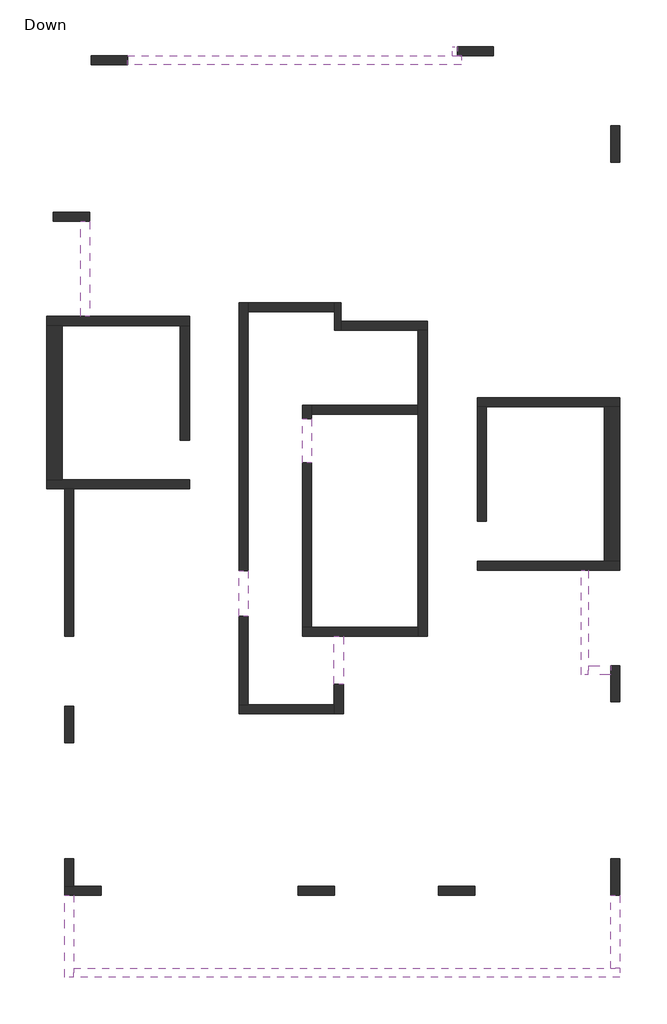
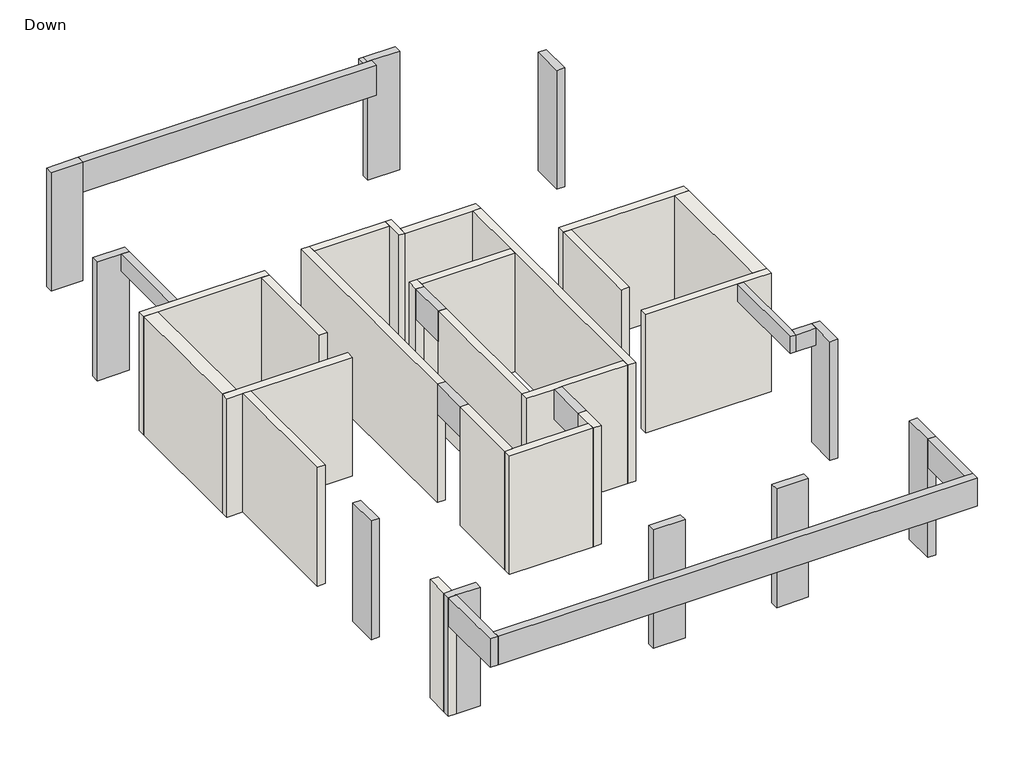
# One storey: 22 walls, 11 beams, 10 columns.
"""IFC4 building model written with IfcOpenShell, lengths in millimetres."""

import ifcopenshell
import ifcopenshell.guid

model = None  # the IFC model being written
_history = None  # IfcOwnerHistory: only IFC2X3 demands one
_inside = {}  # id of a spatial element -> (the spatial element, [elements in it])
_under = {}  # id of a project, library or spatial element -> (it, [spatial elements below it])
_declared = {}  # id of a project -> (the project, [libraries it declares])
_typed = {}  # id of a type object -> (the type object, [elements of that type])
_made_of = {}  # id of a material, layer set ... -> (it, [elements and type objects made of it])


def new_model(schema):
    """Start an empty IFC model of exactly this schema.

    Asked for "IFC4X3", IfcOpenShell would pick the latest addendum, in which some entities
    have other attributes; the version numbers below select the first issue.
    IFC2X3 requires an IfcOwnerHistory on every rooted entity: one is made here for all.
    """
    global model, _history
    if schema == "IFC4X3":
        model = ifcopenshell.file(schema_version=(4, 3, 0, 0))
    else:
        model = ifcopenshell.file(schema=schema)
    _inside.clear()
    _under.clear()
    _declared.clear()
    _typed.clear()
    _made_of.clear()
    _history = None
    if model.schema == "IFC2X3":
        org = make("IfcOrganization", Name="unknown")
        user = make(
            "IfcPersonAndOrganization",
            ThePerson=make("IfcPerson", FamilyName="unknown"),
            TheOrganization=org,
        )
        app = make(
            "IfcApplication",
            ApplicationDeveloper=org,
            Version="unknown",
            ApplicationFullName="unknown",
            ApplicationIdentifier="unknown",
        )
        _history = make(
            "IfcOwnerHistory",
            OwningUser=user,
            OwningApplication=app,
            ChangeAction="ADDED",
            CreationDate=0,
        )
    return model


def make(cls, **values):
    """One entity of the class cls with the attributes given. An attribute that is None is left unset."""
    return model.create_entity(
        cls, **{name: value for name, value in values.items() if value is not None}
    )


def rooted(cls, **values):
    """An entity with a GlobalId (a new one), such as an element, a storey or a relation."""
    return make(cls, GlobalId=ifcopenshell.guid.new(), OwnerHistory=_history, **values)


def si_unit(unit_type, name, prefix=None):
    """IfcSIUnit, for example si_unit("LENGTHUNIT", "METRE", prefix="MILLI")."""
    return make("IfcSIUnit", UnitType=unit_type, Prefix=prefix, Name=name)


def assignment(units):
    """IfcUnitAssignment: the units of a project."""
    return None if units is None else make("IfcUnitAssignment", Units=units)


def point(xyz):
    """IfcCartesianPoint."""
    return None if xyz is None else make("IfcCartesianPoint", Coordinates=xyz)


def direction(xyz):
    """IfcDirection."""
    return None if xyz is None else make("IfcDirection", DirectionRatios=xyz)


def frame(location, z_axis=None, x_axis=None):
    """IfcAxis2Placement3D, a coordinate frame: its origin and axes. An axis left out is left unset."""
    return make(
        "IfcAxis2Placement3D",
        Location=point(location),
        Axis=direction(z_axis),
        RefDirection=direction(x_axis),
    )


def origin():
    """The frame at (0, 0, 0) with its axes left unset."""
    return frame((0.0, 0.0, 0.0))


def place(relative_to, where):
    """IfcLocalPlacement: puts the frame where relative to a parent placement (None: the world)."""
    return make(
        "IfcLocalPlacement", PlacementRelTo=relative_to, RelativePlacement=where
    )


def context(
    kind, dimensions, precision=None, world=None, true_north=None, identifier=None
):
    """IfcGeometricRepresentationContext, for example the 3D "Model" context."""
    return make(
        "IfcGeometricRepresentationContext",
        ContextIdentifier=identifier,
        ContextType=kind,
        CoordinateSpaceDimension=dimensions,
        Precision=precision,
        WorldCoordinateSystem=world,
        TrueNorth=true_north,
    )


def project(units=None, contexts=None):
    """IfcProject with its units and contexts."""
    return rooted(
        "IfcProject",
        Name="project",
        RepresentationContexts=contexts,
        UnitsInContext=assignment(units),
    )


def spatial(cls, under=None, at=None, **own):
    """A site, building, storey or space (cls), placed at a placement, below another one or the project."""
    s = rooted(cls, ObjectPlacement=at, **own)
    if under is not None:
        _under.setdefault(under.id(), (under, []))[1].append(s)
    return s


def polyline(points):
    """IfcPolyline through the points."""
    return make("IfcPolyline", Points=[point(p) for p in points])


def outline(outer, holes=None, kind="AREA"):
    """IfcArbitraryClosedProfileDef: a profile drawn as a closed curve; with holes, ...WithVoids."""
    if holes is None:
        return make("IfcArbitraryClosedProfileDef", ProfileType=kind, OuterCurve=outer)
    return make(
        "IfcArbitraryProfileDefWithVoids",
        ProfileType=kind,
        OuterCurve=outer,
        InnerCurves=holes,
    )


def extrude(swept, where, along, depth):
    """IfcExtrudedAreaSolid: the profile swept, set in the frame where, extruded along a direction by depth."""
    return make(
        "IfcExtrudedAreaSolid",
        SweptArea=swept,
        Position=where,
        ExtrudedDirection=direction(along),
        Depth=depth,
    )


def faces_of(points, faces, orient=None, outer=None):
    """IfcFace entities. A face is a list of loops; a loop is a list of indices into points, from 0.

    orient and outer hold one flag for each loop. By default every Orientation is true, the
    first loop of a face is its IfcFaceOuterBound and the others are IfcFaceBound.
    """
    made = []
    for i, loops in enumerate(faces):
        bounds = []
        for j, loop in enumerate(loops):
            is_outer = j == 0 if outer is None else outer[i][j]
            bounds.append(
                make(
                    "IfcFaceOuterBound" if is_outer else "IfcFaceBound",
                    Bound=make("IfcPolyLoop", Polygon=[points[k] for k in loop]),
                    Orientation=True if orient is None else orient[i][j],
                )
            )
        made.append(make("IfcFace", Bounds=bounds))
    return made


def faceted_brep(points, faces, orient=None, outer=None, voids=None):
    """IfcFacetedBrep: a solid bounded by flat faces; with voids (closed shells), ...WithVoids."""
    shared = [point(p) for p in points]
    hull = make("IfcClosedShell", CfsFaces=faces_of(shared, faces, orient, outer))
    if voids is None:
        return make("IfcFacetedBrep", Outer=hull)
    return make(
        "IfcFacetedBrepWithVoids",
        Outer=hull,
        Voids=[
            make(cls, CfsFaces=faces_of(shared, fs, o, b)) for cls, fs, o, b in voids
        ],
    )


def shape(context_of_items, identifier, shape_type, items):
    """IfcShapeRepresentation: the items that make up one representation, for example the "Body"."""
    return make(
        "IfcShapeRepresentation",
        ContextOfItems=context_of_items,
        RepresentationIdentifier=identifier,
        RepresentationType=shape_type,
        Items=items,
    )


def made_of(thing, what):
    """Note that an element or type object is made of a material, layer set ...; save() writes the relation."""
    if what is not None:
        _made_of.setdefault(what.id(), (what, []))[1].append(thing)
    return thing


def element(
    cls,
    number,
    at=None,
    inside=None,
    cuts=None,
    type_object=None,
    material=None,
    context=None,
    identifier="Body",
    shape_type=None,
    held_by="IfcProductDefinitionShape",
    body=None,
    shapes=None,
    **own,
):
    """One element of the class cls, such as IfcWall. Its Tag is "e" and its number.

    at: its placement. inside: the storey or other place that contains it. cuts: it is an
    opening in that element (IfcRelVoidsElement). A single representation is given by context,
    identifier, shape_type and body (its items); several are given by shapes. held_by: the class
    of the entity that holds the representations. save() writes the other relations.
    """
    e = rooted(cls, Tag="e%d" % number, ObjectPlacement=at, **own)
    if body is not None:
        shapes = [shape(context, identifier, shape_type, body)]
    if shapes is not None:
        e.Representation = make(held_by, Representations=shapes)
    if inside is not None:
        _inside.setdefault(inside.id(), (inside, []))[1].append(e)
    if cuts is not None:
        rooted(
            "IfcRelVoidsElement", RelatingBuildingElement=cuts, RelatedOpeningElement=e
        )
    if type_object is not None:
        _typed.setdefault(type_object.id(), (type_object, []))[1].append(e)
    return made_of(e, material)


def aggregate(whole, parts):
    """IfcRelAggregates: a whole, such as a stair, and the parts it consists of."""
    return rooted("IfcRelAggregates", RelatingObject=whole, RelatedObjects=parts)


def save(model, path):
    """Write the relations noted so far, then the file.

    IfcRelAggregates (storeys below a building ...), IfcRelContainedInSpatialStructure (elements
    in a storey), IfcRelDefinesByType, IfcRelAssociatesMaterial and IfcRelDeclares: one each for
    every whole, place, type object, material and project.
    """
    for whole, parts in _under.values():
        aggregate(whole, parts)
    for where, things in _inside.values():
        rooted(
            "IfcRelContainedInSpatialStructure",
            RelatedElements=things,
            RelatingStructure=where,
        )
    for kind, things in _typed.values():
        rooted("IfcRelDefinesByType", RelatedObjects=things, RelatingType=kind)
    for what, things in _made_of.values():
        rooted("IfcRelAssociatesMaterial", RelatedObjects=things, RelatingMaterial=what)
    for by, libraries in _declared.values():
        rooted("IfcRelDeclares", RelatingContext=by, RelatedDefinitions=libraries)
    model.write(path)


model = new_model("IFC4")

# Units and contexts
model_context = context("Model", 3, world=origin())
ifc_project = project(units=[si_unit("LENGTHUNIT", "METRE", prefix="MILLI")], contexts=[model_context])

# Site, building, storey
site = spatial("IfcSite", under=ifc_project)
building = spatial("IfcBuilding", under=site)
storey = spatial("IfcBuildingStorey", under=building, Name="Down", Elevation=0.0)

# Beams
placement = place(None, origin())
element("IfcBeam", 1, ObjectType="Concrete Rectengular Beam : 15/45", at=placement, inside=storey, context=model_context, shape_type="Brep", body=[
    faceted_brep([(-8943.1419846, 24273.2318976, 3150.0), (-9093.1419846, 24273.2318976, 3150.0), (-9093.1419846, 21971.29434, 3150.0), (-8943.1419846, 21971.29434, 3150.0), (-8943.1419846, 22171.29434, 3150.0), (-9093.1419846, 24273.2318976, 2920.0), (-9093.1419846, 24273.2318976, 2700.0), (-9093.1419846, 21971.29434, 2700.0), (-9093.1419846, 21971.29434, 2920.0), (-8943.1419846, 24273.2318976, 2700.0), (-8943.1419846, 22171.4624057, 2700.0), (-8943.1419846, 22171.29434, 2700.0), (-8943.1419846, 21971.29434, 2700.0), (-8943.1419846, 24273.2318976, 2850.0), (-8943.1419846, 21971.29434, 2920.0)], [[[0, 1, 2, 3, 4]], [[2, 1, 5, 6, 7, 8]], [[6, 9, 10, 11, 12, 7]], [[9, 13, 0, 4, 3, 14, 12, 11, 10]], [[1, 0, 13, 9, 6, 5]], [[3, 2, 8, 7, 12, 14]]]),
])
element("IfcBeam", 2, ObjectType="Concrete Rectengular Beam : 20/45", at=placement, inside=storey, context=model_context, shape_type="Brep", body=[
    faceted_brep([(-19934.1305711, 31959.1185492, 3150.0), (-20134.1305711, 31959.1185492, 3150.0), (-20134.1305711, 29864.251036, 3150.0), (-19934.1305711, 29864.251036, 3150.0), (-20134.1305711, 31959.1185492, 2850.0), (-20134.1305711, 31959.1185492, 2700.0), (-20134.1305711, 29864.251036, 2700.0), (-20134.1305711, 29864.251036, 2850.0), (-19934.1305711, 31959.1185492, 2700.0), (-19934.1305711, 29864.251036, 2700.0), (-19934.1305711, 29864.251036, 2920.0), (-19934.1305711, 31959.1185492, 2920.0)], [[[0, 1, 2, 3]], [[1, 4, 5, 6, 7, 2]], [[5, 8, 9, 6]], [[0, 3, 10, 9, 8, 11]], [[1, 0, 11, 8, 5, 4]], [[3, 2, 7, 6, 9, 10]]]),
])
element("IfcBeam", 3, ObjectType="Concrete Rectengular Beam : 20/45", at=placement, inside=storey, context=model_context, shape_type="Brep", body=[
    faceted_brep([(-8445.045869, 21971.29434, 3150.0), (-8445.045869, 22171.29434, 3150.0), (-8943.1419846, 22171.29434, 3150.0), (-8943.1419846, 21971.29434, 3150.0), (-8445.045869, 22171.29434, 2700.0), (-8943.1419846, 22171.29434, 2700.0), (-8445.045869, 21971.29434, 2700.0), (-8943.1419846, 21971.29434, 2700.0), (-8445.045869, 21971.29434, 2920.0)], [[[0, 1, 2, 3]], [[1, 4, 5, 2]], [[4, 6, 7, 5]], [[6, 8, 0, 3, 7]], [[1, 0, 8, 6, 4]], [[3, 2, 5, 7]]]),
])
element("IfcBeam", 4, ObjectType="Concrete Rectengular Beam : 20/75", at=placement, inside=storey, context=model_context, shape_type="Brep", body=[
    faceted_brep([(-20285.7922608, 17115.8692988, 3150.0), (-20485.7922608, 17115.8692988, 3150.0), (-20485.7922608, 15302.6614945, 3150.0), (-20285.7922608, 15302.6614945, 3150.0), (-20285.7922608, 15502.6614945, 3150.0), (-20485.7922608, 15302.6614945, 2400.0), (-20485.7922608, 17115.8692988, 2400.0), (-20285.7922608, 17115.8692988, 2400.0), (-20285.7922608, 15502.6614945, 2400.0), (-20285.7922608, 15302.6614945, 2400.0), (-20285.7922608, 17115.8692988, 2920.0)], [[[0, 1, 2, 3, 4]], [[5, 2, 1, 6]], [[6, 7, 8, 9, 5]], [[3, 9, 8, 7, 10, 0, 4]], [[1, 0, 10, 7, 6]], [[3, 2, 5, 9]]]),
])
element("IfcBeam", 5, ObjectType="Concrete Rectengular Beam : 20/75", at=placement, inside=storey, context=model_context, shape_type="Brep", body=[
    faceted_brep([(-8245.045869, 15302.6614945, 3150.0), (-8245.045869, 15502.6614945, 3150.0), (-8445.045869, 15502.6614945, 3150.0), (-20285.7922608, 15502.6614945, 3150.0), (-20285.7922608, 15302.6614945, 3150.0), (-8245.045869, 15302.6614945, 2400.0), (-20285.7922608, 15302.6614945, 2400.0), (-8245.045869, 15502.6614945, 2400.0), (-20285.7922608, 15502.6614945, 2400.0), (-8445.045869, 15502.6614945, 2400.0), (-20285.7922608, 15502.6614945, 2920.0)], [[[0, 1, 2, 3, 4]], [[5, 0, 4, 6]], [[7, 5, 6, 8, 9]], [[1, 7, 9, 8, 10, 3, 2]], [[4, 3, 10, 8, 6]], [[1, 0, 5, 7]]]),
])
element("IfcBeam", 6, ObjectType="Concrete Rectengular Beam : 20/75", at=placement, inside=storey, context=model_context, shape_type="Brep", body=[
    faceted_brep([(-8245.045869, 17114.2549976, 3150.0), (-8445.045869, 17114.2549976, 3150.0), (-8445.045869, 15502.6614945, 3150.0), (-8245.045869, 15502.6614945, 3150.0), (-8245.045869, 17114.2549976, 2400.0), (-8245.045869, 15502.6614945, 2400.0), (-8445.045869, 17114.2549976, 2400.0), (-8445.045869, 15502.6614945, 2400.0), (-8445.045869, 17114.2549976, 2920.0), (-8445.045869, 15502.6614945, 2920.0)], [[[0, 1, 2, 3]], [[4, 0, 3, 5]], [[6, 4, 5, 7]], [[2, 1, 8, 6, 7, 9]], [[1, 0, 4, 6, 8]], [[3, 2, 9, 7, 5]]]),
])
element("IfcBeam", 7, ObjectType="Concrete Rectengular Beam : 20/80", at=placement, inside=storey, context=model_context, shape_type="Brep", body=[
    faceted_brep([(-11741.5564046, 35608.8121294, 3150.0), (-11741.5564046, 35408.8121294, 3150.0), (-11741.5564046, 35408.8121294, 2920.0), (-11741.5564046, 35408.8121294, 2350.0), (-11741.5564046, 35608.8121294, 2350.0), (-11741.5564046, 35608.8121294, 2920.0), (-11742.9937266, 35608.8121294, 3150.0), (-11942.9937266, 35608.8121294, 3150.0), (-19101.5564046, 35608.8121294, 3150.0), (-19101.5564046, 35408.8121294, 3150.0), (-19101.5564046, 35408.8121294, 2920.0), (-19101.5564046, 35408.8121294, 2350.0), (-19101.5564046, 35608.8121294, 2350.0), (-11942.9937266, 35608.8121294, 2350.0), (-11742.9937266, 35608.8121294, 2350.0)], [[[0, 1, 2, 3, 4, 5]], [[1, 0, 6, 7, 8, 9]], [[1, 9, 10, 11, 3, 2]], [[4, 3, 11, 12, 13, 14]], [[12, 8, 7, 6, 0, 5, 4, 14, 13]], [[9, 8, 12, 11, 10]]]),
])
element("IfcBeam", 8, ObjectType="Concrete Rectengular Beam : 20/80", at=placement, inside=storey, context=model_context, shape_type="SweptSolid", body=[
    extrude(outline(polyline([(-11833.3239157, 35608.9801951), (-11742.9937266, 35608.9801951), (-11742.9937266, 35608.8121294), (-11942.9937266, 35608.8121294), (-11942.9937266, 35808.8121294), (-11833.3239157, 35808.8121294), (-11833.3239157, 35608.9801951)])), frame((0.0, 0.0, 2350.0), z_axis=(0.0, 0.0, 1.0), x_axis=(1.0, 0.0, 0.0)), (0.0, 0.0, 1.0), 800.0),
])
element("IfcBeam", 9, ObjectType="Concrete Rectengular Beam : 20/80", at=placement, inside=storey, context=model_context, shape_type="Brep", body=[
    faceted_brep([(-16642.902761, 24264.0058702, 3150.0), (-16442.902761, 24264.0058702, 3150.0), (-16442.902761, 24264.0058702, 2350.0), (-16642.902761, 24264.0058702, 2350.0), (-16642.902761, 24264.0058702, 2920.0), (-16642.902761, 23263.128057, 2350.0), (-16442.902761, 23263.128057, 2350.0), (-16442.902761, 23263.128057, 3150.0), (-16642.902761, 23263.128057, 3150.0), (-16642.902761, 23263.128057, 2920.0)], [[[0, 1, 2, 3, 4]], [[5, 6, 7, 8, 9]], [[1, 0, 8, 7]], [[2, 1, 7, 6]], [[3, 2, 6, 5]], [[8, 0, 4, 3, 5, 9]]]),
])
element("IfcBeam", 10, ObjectType="Concrete Rectengular Beam : 20/80", at=placement, inside=storey, context=model_context, shape_type="Brep", body=[
    faceted_brep([(-15041.6888164, 27611.1233031, 2350.0), (-15241.6888164, 27611.1233031, 2350.0), (-15241.6888164, 27611.1233031, 2920.0), (-15241.6888164, 27611.1233031, 3150.0), (-15046.6888164, 27611.1233031, 3150.0), (-15046.6888164, 27611.1233031, 2920.0), (-15041.6888164, 27611.1233031, 2920.0), (-15241.6888164, 26638.171559, 2350.0), (-15041.6888164, 26638.171559, 2350.0), (-15041.6888164, 26638.171559, 2920.0), (-15046.6888164, 26638.171559, 2920.0), (-15046.6888164, 26638.171559, 3150.0), (-15241.6888164, 26638.171559, 3150.0), (-15241.6888164, 26638.171559, 2920.0)], [[[0, 1, 2, 3, 4, 5, 6]], [[7, 8, 9, 10, 11, 12, 13]], [[3, 12, 11, 4]], [[8, 0, 6, 9]], [[1, 0, 8, 7]], [[12, 3, 2, 1, 7, 13]], [[5, 10, 9, 6]], [[10, 5, 4, 11]]]),
])
element("IfcBeam", 11, ObjectType="Concrete Rectengular Beam : 20/80", at=placement, inside=storey, context=model_context, shape_type="Brep", body=[
    faceted_brep([(-14543.2190847, 21764.1541281, 2350.0), (-14343.2190847, 21764.1541281, 2350.0), (-14343.2190847, 21764.1541281, 2920.0), (-14343.2190847, 21764.1541281, 3150.0), (-14543.2190847, 21764.1541281, 3150.0), (-14543.2190847, 21764.1541281, 2920.0), (-14343.2190847, 22813.9119334, 3150.0), (-14543.2190847, 22813.9119334, 3150.0), (-14343.2190847, 22813.9119334, 2350.0), (-14343.2190847, 22813.9119334, 2920.0), (-14543.2190847, 22813.9119334, 2350.0), (-14543.2190847, 22813.9119334, 2920.0)], [[[0, 1, 2, 3, 4, 5]], [[4, 3, 6, 7]], [[6, 3, 2, 1, 8, 9]], [[1, 0, 10, 8]], [[4, 7, 11, 10, 0, 5]], [[7, 6, 9, 8, 10, 11]]]),
])

# Columns
element("IfcColumn", 12, ObjectType="Concrete Rectengular Column : 20/80", at=placement, inside=storey, context=model_context, shape_type="Brep", body=[
    faceted_brep([(-19901.5564046, 35608.8121294, 0.0), (-19101.5564046, 35608.8121294, 0.0), (-19101.5564046, 35408.8121294, 0.0), (-19901.5564046, 35408.8121294, 0.0), (-19901.5564046, 35608.8121294, 3150.0), (-19101.5564046, 35608.8121294, 3150.0), (-19901.5564046, 35608.8121294, 2920.0), (-19101.5564046, 35408.8121294, 3150.0), (-19901.5564046, 35408.8121294, 3150.0), (-19901.5564046, 35408.8121294, 2920.0)], [[[0, 1, 2, 3]], [[4, 5, 1, 0, 6]], [[5, 7, 2, 1]], [[7, 8, 9, 3, 2]], [[8, 4, 6, 0, 3, 9]], [[4, 8, 7, 5]]]),
])
element("IfcColumn", 13, ObjectType="Concrete Rectengular Column : 20/80", at=placement, inside=storey, context=model_context, shape_type="Brep", body=[
    faceted_brep([(-11833.3239157, 35808.9801951, 0.0), (-11033.3239157, 35808.9801951, 0.0), (-11033.3239157, 35608.9801951, 0.0), (-11833.3239157, 35608.9801951, 0.0), (-11833.3239157, 35808.9801951, 3150.0), (-11033.3239157, 35808.9801951, 3150.0), (-11033.3239157, 35808.9801951, 2920.0), (-11033.3239157, 35608.9801951, 3150.0), (-11033.3239157, 35608.9801951, 2920.0), (-11741.5564046, 35608.9801951, 3150.0), (-11833.3239157, 35608.9801951, 3150.0)], [[[0, 1, 2, 3]], [[4, 5, 6, 1, 0]], [[5, 7, 8, 2, 1, 6]], [[7, 9, 10, 3, 2, 8]], [[10, 4, 0, 3]], [[4, 10, 9, 7, 5]]]),
])
element("IfcColumn", 14, ObjectType="Concrete Rectengular Column : 20/80", at=placement, inside=storey, context=model_context, shape_type="Brep", body=[
    faceted_brep([(-8445.045869, 33260.248461, 0.0), (-8445.045869, 34060.248461, 0.0), (-8245.045869, 34060.248461, 0.0), (-8245.045869, 33260.248461, 0.0), (-8445.045869, 33260.248461, 3150.0), (-8445.045869, 34060.248461, 3150.0), (-8445.045869, 34060.248461, 2920.0), (-8445.045869, 33260.248461, 2920.0), (-8245.045869, 34060.248461, 3150.0), (-8245.045869, 34060.248461, 2920.0), (-8245.045869, 33260.248461, 3150.0), (-8245.045869, 33260.248461, 2920.0)], [[[0, 1, 2, 3]], [[4, 5, 6, 1, 0, 7]], [[5, 8, 9, 2, 1, 6]], [[8, 10, 11, 3, 2, 9]], [[10, 4, 7, 0, 3, 11]], [[4, 10, 8, 5]]]),
])
element("IfcColumn", 15, ObjectType="Concrete Rectengular Column : 20/80", at=placement, inside=storey, context=model_context, shape_type="Brep", body=[
    faceted_brep([(-8445.045869, 21371.4624057, 0.0), (-8445.045869, 22171.4624057, 0.0), (-8245.045869, 22171.4624057, 0.0), (-8245.045869, 21371.4624057, 0.0), (-8445.045869, 21371.4624057, 3150.0), (-8445.045869, 21971.29434, 3150.0), (-8445.045869, 22171.4624057, 3150.0), (-8445.045869, 21371.4624057, 2920.0), (-8245.045869, 22171.4624057, 3150.0), (-8245.045869, 22171.4624057, 2850.0), (-8245.045869, 22171.4624057, 2700.0), (-8245.045869, 21371.4624057, 3150.0), (-8245.045869, 21371.4624057, 2920.0)], [[[0, 1, 2, 3]], [[4, 5, 6, 1, 0, 7]], [[6, 8, 9, 10, 2, 1]], [[8, 11, 12, 3, 2, 10, 9]], [[11, 4, 7, 0, 3, 12]], [[4, 11, 8, 6, 5]]]),
])
element("IfcColumn", 16, ObjectType="Concrete Rectengular Column : 20/80", at=placement, inside=storey, context=model_context, shape_type="Brep", body=[
    faceted_brep([(-8445.045869, 17114.2549976, 0.0), (-8445.045869, 17914.2549976, 0.0), (-8245.045869, 17914.2549976, 0.0), (-8245.045869, 17114.2549976, 0.0), (-8445.045869, 17114.2549976, 3150.0), (-8445.045869, 17914.2549976, 3150.0), (-8445.045869, 17914.2549976, 2920.0), (-8245.045869, 17914.2549976, 3150.0), (-8245.045869, 17914.2549976, 2920.0), (-8245.045869, 17114.2549976, 3150.0)], [[[0, 1, 2, 3]], [[4, 5, 6, 1, 0]], [[5, 7, 8, 2, 1, 6]], [[7, 9, 3, 2, 8]], [[9, 4, 0, 3]], [[4, 9, 7, 5]]]),
])
element("IfcColumn", 17, ObjectType="Concrete Rectengular Column : 20/80", at=placement, inside=storey, context=model_context, shape_type="Brep", body=[
    faceted_brep([(-12242.9937266, 17316.0748491, 0.0), (-11442.9937266, 17316.0748491, 0.0), (-11442.9937266, 17116.0748491, 0.0), (-12242.9937266, 17116.0748491, 0.0), (-12242.9937266, 17316.0748491, 3150.0), (-11442.9937266, 17316.0748491, 3150.0), (-11442.9937266, 17316.0748491, 2920.0), (-12242.9937266, 17316.0748491, 2920.0), (-11442.9937266, 17116.0748491, 3150.0), (-11442.9937266, 17116.0748491, 2920.0), (-12242.9937266, 17116.0748491, 3150.0), (-12242.9937266, 17116.0748491, 2920.0)], [[[0, 1, 2, 3]], [[4, 5, 6, 1, 0, 7]], [[5, 8, 9, 2, 1, 6]], [[8, 10, 11, 3, 2, 9]], [[10, 4, 7, 0, 3, 11]], [[4, 10, 8, 5]]]),
])
element("IfcColumn", 18, ObjectType="Concrete Rectengular Column : 20/80", at=placement, inside=storey, context=model_context, shape_type="Brep", body=[
    faceted_brep([(-15341.7353646, 17316.0748491, 0.0), (-14541.7353646, 17316.0748491, 0.0), (-14541.7353646, 17116.0748491, 0.0), (-15341.7353646, 17116.0748491, 0.0), (-15341.7353646, 17316.0748491, 3150.0), (-14541.7353646, 17316.0748491, 3150.0), (-14541.7353646, 17316.0748491, 2920.0), (-15341.7353646, 17316.0748491, 2920.0), (-14541.7353646, 17116.0748491, 3150.0), (-14541.7353646, 17116.0748491, 2920.0), (-15341.7353646, 17116.0748491, 3150.0), (-15341.7353646, 17116.0748491, 2920.0)], [[[0, 1, 2, 3]], [[4, 5, 6, 1, 0, 7]], [[5, 8, 9, 2, 1, 6]], [[8, 10, 11, 3, 2, 9]], [[10, 4, 7, 0, 3, 11]], [[4, 10, 8, 5]]]),
])
element("IfcColumn", 19, ObjectType="Concrete Rectengular Column : 20/80", at=placement, inside=storey, context=model_context, shape_type="Brep", body=[
    faceted_brep([(-20485.7922608, 17316.0748491, 0.0), (-20285.7922608, 17316.0748491, 0.0), (-19685.7922608, 17316.0748491, 0.0), (-19685.7922608, 17116.0748491, 0.0), (-20285.7922608, 17116.0748491, 0.0), (-20485.7922608, 17116.0748491, 0.0), (-20485.7922608, 17316.0748491, 3150.0), (-20285.7922608, 17316.0748491, 3150.0), (-19685.7922608, 17316.0748491, 3150.0), (-19685.7922608, 17316.0748491, 2920.0), (-19685.7922608, 17116.0748491, 3150.0), (-19685.7922608, 17116.0748491, 2920.0), (-20285.7922608, 17116.0748491, 3150.0), (-20485.7922608, 17116.0748491, 3150.0)], [[[0, 1, 2, 3, 4, 5]], [[6, 7, 8, 9, 2, 1, 0]], [[8, 10, 11, 3, 2, 9]], [[10, 12, 13, 5, 4, 3, 11]], [[13, 6, 0, 5]], [[6, 13, 12, 10, 8, 7]]]),
])
element("IfcColumn", 20, ObjectType="Concrete Rectengular Column : 20/80", at=placement, inside=storey, context=model_context, shape_type="Brep", body=[
    faceted_brep([(-20485.7922608, 20472.3204112, 0.0), (-20485.7922608, 21272.3204112, 0.0), (-20285.7922608, 21272.3204112, 0.0), (-20285.7922608, 20472.3204112, 0.0), (-20485.7922608, 20472.3204112, 3150.0), (-20485.7922608, 21272.3204112, 3150.0), (-20485.7922608, 20472.3204112, 2920.0), (-20285.7922608, 21272.3204112, 3150.0), (-20285.7922608, 21272.3204112, 2920.0), (-20285.7922608, 20472.3204112, 3150.0), (-20285.7922608, 20472.3204112, 2920.0)], [[[0, 1, 2, 3]], [[4, 5, 1, 0, 6]], [[5, 7, 8, 2, 1]], [[7, 9, 10, 3, 2, 8]], [[9, 4, 6, 0, 3, 10]], [[4, 9, 7, 5]]]),
])
element("IfcColumn", 21, ObjectType="Concrete Rectengular Column : 20/80", at=placement, inside=storey, context=model_context, shape_type="Brep", body=[
    faceted_brep([(-20734.1305711, 32159.1185492, 0.0), (-19934.1305711, 32159.1185492, 0.0), (-19934.1305711, 31959.1185492, 0.0), (-20734.1305711, 31959.1185492, 0.0), (-20734.1305711, 32159.1185492, 3150.0), (-19934.1305711, 32159.1185492, 3150.0), (-19934.1305711, 32159.1185492, 2920.0), (-20734.1305711, 32159.1185492, 2700.0), (-20734.1305711, 32159.1185492, 2850.0), (-20734.1305711, 32159.1185492, 2920.0), (-19934.1305711, 31959.1185492, 3150.0), (-20734.1305711, 31959.1185492, 3150.0), (-20734.1305711, 31959.1185492, 2850.0), (-20734.1305711, 31959.1185492, 2700.0)], [[[0, 1, 2, 3]], [[4, 5, 6, 1, 0, 7, 8, 9]], [[5, 10, 2, 1, 6]], [[10, 11, 12, 13, 3, 2]], [[11, 4, 9, 8, 7, 0, 3, 13, 12]], [[4, 11, 10, 5]]]),
])

# Walls
element("IfcWall", 22, ObjectType="15", at=placement, inside=storey, context=model_context, shape_type="Brep", body=[
    faceted_brep([(-14392.0990768, 29561.6748888, 0.0), (-14392.0990768, 29761.6748888, 0.0), (-14392.0990768, 30162.1790859, 0.0), (-14392.0990768, 30162.1790859, 2920.0), (-14392.0990768, 30162.1790859, 3150.0), (-14392.0990768, 29761.6748888, 3150.0), (-14392.0990768, 29561.6748888, 3150.0), (-14392.0990768, 29561.6748888, 2920.0), (-14542.0990768, 29561.6748888, 0.0), (-14542.0990768, 29561.6748888, 2920.0), (-14542.0990768, 29561.6748888, 3150.0), (-14542.0990768, 29962.1790859, 3150.0), (-14542.0990768, 30162.1790859, 3150.0), (-14542.0990768, 30162.1790859, 0.0), (-14542.0990768, 29962.1790859, 0.0)], [[[0, 1, 2, 3, 4, 5, 6, 7]], [[8, 9, 10, 11, 12, 13, 14]], [[2, 1, 0, 8, 14, 13]], [[6, 5, 4, 12, 11, 10]], [[4, 3, 2, 13, 12]], [[0, 7, 6, 10, 9, 8]]]),
])
element("IfcWall", 23, ObjectType="20", at=placement, inside=storey, context=model_context, shape_type="Brep", body=[
    faceted_brep([(-20886.1283922, 29664.251036, 0.0), (-20536.1283922, 29664.251036, 0.0), (-17936.892461, 29664.251036, 0.0), (-17736.892461, 29664.251036, 0.0), (-17736.892461, 29664.251036, 3150.0), (-17936.892461, 29664.251036, 3150.0), (-20536.1283922, 29664.251036, 3150.0), (-20886.1283922, 29664.251036, 3150.0), (-20886.1283922, 29864.251036, 0.0), (-20886.1283922, 29864.251036, 2700.0), (-20886.1283922, 29864.251036, 2850.0), (-20886.1283922, 29864.251036, 3150.0), (-19934.1305711, 29864.251036, 3150.0), (-17736.892461, 29864.251036, 3150.0), (-17736.892461, 29864.251036, 2920.0), (-17736.892461, 29864.251036, 0.0)], [[[0, 1, 2, 3, 4, 5, 6, 7]], [[8, 9, 10, 11, 12, 13, 14, 15]], [[3, 2, 1, 0, 8, 15]], [[7, 6, 5, 4, 13, 12, 11]], [[4, 3, 15, 14, 13]], [[0, 7, 11, 10, 9, 8]]]),
])
element("IfcWall", 24, ObjectType="20", at=placement, inside=storey, context=model_context, shape_type="Brep", body=[
    faceted_brep([(-17936.892461, 29664.251036, 0.0), (-17936.892461, 27140.9157719, 0.0), (-17936.892461, 27140.9157719, 2920.0), (-17936.892461, 27140.9157719, 3150.0), (-17936.892461, 29664.251036, 3150.0), (-17936.892461, 29664.251036, 2920.0), (-17736.892461, 29664.251036, 0.0), (-17736.892461, 29664.251036, 3150.0), (-17736.892461, 27140.9157719, 3150.0), (-17736.892461, 27140.9157719, 2920.0), (-17736.892461, 27140.9157719, 0.0), (-17926.892461, 27140.9157719, 3150.0)], [[[0, 1, 2, 3, 4, 5]], [[6, 7, 8, 9, 10]], [[1, 0, 6, 10]], [[3, 2, 1, 10, 9, 8, 11]], [[4, 3, 11, 8, 7]], [[0, 5, 4, 7, 6]]]),
])
element("IfcWall", 25, ObjectType="20", at=placement, inside=storey, context=model_context, shape_type="Brep", body=[
    faceted_brep([(-17736.892461, 26263.2318976, 0.0), (-20536.1283922, 26263.2318976, 0.0), (-20886.1283922, 26263.2318976, 0.0), (-20886.1283922, 26263.2318976, 3150.0), (-20536.1283922, 26263.2318976, 3150.0), (-17926.892461, 26263.2318976, 3150.0), (-17736.892461, 26263.2318976, 3150.0), (-17736.892461, 26263.2318976, 2920.0), (-17736.892461, 26063.2318976, 0.0), (-17736.892461, 26063.2318976, 2920.0), (-17736.892461, 26063.2318976, 3150.0), (-20287.9482438, 26063.2318976, 3150.0), (-20487.9482438, 26063.2318976, 3150.0), (-20886.1283922, 26063.2318976, 3150.0), (-20886.1283922, 26063.2318976, 0.0), (-20487.9482438, 26063.2318976, 0.0), (-20287.9482438, 26063.2318976, 0.0)], [[[0, 1, 2, 3, 4, 5, 6, 7]], [[8, 9, 10, 11, 12, 13, 14, 15, 16]], [[2, 1, 0, 8, 16, 15, 14]], [[6, 5, 4, 3, 13, 12, 11, 10]], [[0, 7, 6, 10, 9, 8]], [[3, 2, 14, 13]]]),
])
element("IfcWall", 26, ObjectType="20", at=placement, inside=storey, context=model_context, shape_type="Brep", body=[
    faceted_brep([(-20487.9482438, 26063.2318976, 0.0), (-20487.9482438, 22813.9119334, 0.0), (-20487.9482438, 22813.9119334, 2920.0), (-20487.9482438, 22813.9119334, 3150.0), (-20487.9482438, 26063.2318976, 3150.0), (-20287.9482438, 26063.2318976, 0.0), (-20287.9482438, 26063.2318976, 2920.0), (-20287.9482438, 26063.2318976, 3150.0), (-20287.9482438, 22813.9119334, 3150.0), (-20287.9482438, 22813.9119334, 2920.0), (-20287.9482438, 22813.9119334, 0.0)], [[[0, 1, 2, 3, 4]], [[5, 6, 7, 8, 9, 10]], [[1, 0, 5, 10]], [[3, 2, 1, 10, 9, 8]], [[4, 3, 8, 7]], [[0, 4, 7, 6, 5]]]),
])
element("IfcWall", 27, ObjectType="20", at=placement, inside=storey, context=model_context, shape_type="Brep", body=[
    faceted_brep([(-20485.7922608, 17115.8692988, 0.0), (-20485.7922608, 17115.8692988, 2400.0), (-20485.7922608, 17115.8692988, 3150.0), (-20485.7922608, 17116.0748491, 3150.0), (-20485.7922608, 17116.0748491, 0.0), (-20285.7922608, 17115.8692988, 3150.0), (-20285.7922608, 17115.8692988, 2400.0), (-20285.7922608, 17115.8692988, 0.0), (-20285.7922608, 17116.0748491, 0.0), (-20285.7922608, 17116.0748491, 2920.0), (-20285.7922608, 17116.0748491, 3150.0)], [[[0, 1, 2, 3, 4]], [[5, 6, 7, 8, 9, 10]], [[7, 0, 4, 8]], [[2, 1, 0, 7, 6, 5]], [[2, 5, 10, 3]], [[4, 3, 10, 9, 8]]]),
    faceted_brep([(-20485.7922608, 17914.2549976, 3150.0), (-20485.7922608, 17914.2549976, 2920.0), (-20485.7922608, 17914.2549976, 0.0), (-20485.7922608, 17316.0748491, 0.0), (-20485.7922608, 17316.0748491, 3150.0), (-20285.7922608, 17914.2549976, 0.0), (-20285.7922608, 17914.2549976, 2920.0), (-20285.7922608, 17914.2549976, 3150.0), (-20285.7922608, 17316.0748491, 3150.0), (-20285.7922608, 17316.0748491, 2920.0), (-20285.7922608, 17316.0748491, 0.0)], [[[0, 1, 2, 3, 4]], [[5, 6, 7, 8, 9, 10]], [[2, 5, 10, 3]], [[7, 0, 4, 8]], [[2, 1, 0, 7, 6, 5]], [[4, 3, 10, 9, 8]]]),
])
element("IfcWall", 28, ObjectType="20", at=placement, inside=storey, context=model_context, shape_type="Brep", body=[
    faceted_brep([(-14543.2190847, 21764.1541281, 0.0), (-14543.2190847, 21314.7324543, 0.0), (-14543.2190847, 21114.7324543, 0.0), (-14543.2190847, 21114.7324543, 3150.0), (-14543.2190847, 21314.7324543, 3150.0), (-14543.2190847, 21764.1541281, 3150.0), (-14543.2190847, 21764.1541281, 2350.0), (-14343.2190847, 21764.1541281, 0.0), (-14343.2190847, 21764.1541281, 2350.0), (-14343.2190847, 21764.1541281, 3150.0), (-14343.2190847, 21114.7324543, 3150.0), (-14343.2190847, 21114.7324543, 2920.0), (-14343.2190847, 21114.7324543, 0.0)], [[[0, 1, 2, 3, 4, 5, 6]], [[7, 8, 9, 10, 11, 12]], [[2, 1, 0, 7, 12]], [[5, 4, 3, 10, 9]], [[0, 6, 5, 9, 8, 7]], [[3, 2, 12, 11, 10]]]),
])
element("IfcWall", 29, ObjectType="20", at=placement, inside=storey, context=model_context, shape_type="Brep", body=[
    faceted_brep([(-14543.2190847, 21314.7324543, 0.0), (-16442.902761, 21314.7324543, 0.0), (-16642.902761, 21314.7324543, 0.0), (-16642.902761, 21314.7324543, 3150.0), (-16442.902761, 21314.7324543, 3150.0), (-14543.2190847, 21314.7324543, 3150.0), (-14543.2190847, 21314.7324543, 2920.0), (-14543.2190847, 21114.7324543, 0.0), (-14543.2190847, 21114.7324543, 3150.0), (-16642.902761, 21114.7324543, 3150.0), (-16642.902761, 21114.7324543, 2920.0), (-16642.902761, 21114.7324543, 0.0)], [[[0, 1, 2, 3, 4, 5, 6]], [[7, 8, 9, 10, 11]], [[2, 1, 0, 7, 11]], [[5, 4, 3, 9, 8]], [[0, 6, 5, 8, 7]], [[3, 2, 11, 10, 9]]]),
])
element("IfcWall", 30, ObjectType="20", at=placement, inside=storey, context=model_context, shape_type="Brep", body=[
    faceted_brep([(-16442.902761, 21314.7324543, 0.0), (-16442.902761, 23263.128057, 0.0), (-16442.902761, 23263.128057, 2350.0), (-16442.902761, 23263.128057, 3150.0), (-16442.902761, 21314.7324543, 3150.0), (-16442.902761, 21314.7324543, 2920.0), (-16642.902761, 21314.7324543, 0.0), (-16642.902761, 21314.7324543, 3150.0), (-16642.902761, 23263.128057, 3150.0), (-16642.902761, 23263.128057, 2350.0), (-16642.902761, 23263.128057, 0.0)], [[[0, 1, 2, 3, 4, 5]], [[6, 7, 8, 9, 10]], [[1, 0, 6, 10]], [[3, 2, 1, 10, 9, 8]], [[4, 3, 8, 7]], [[0, 5, 4, 7, 6]]]),
])
element("IfcWall", 31, ObjectType="20", at=placement, inside=storey, context=model_context, shape_type="Brep", body=[
    faceted_brep([(-16442.902761, 24264.0058702, 0.0), (-16442.902761, 29962.1790859, 0.0), (-16442.902761, 30162.1790859, 0.0), (-16442.902761, 30162.1790859, 3150.0), (-16442.902761, 29962.1790859, 3150.0), (-16442.902761, 24264.0058702, 3150.0), (-16442.902761, 24264.0058702, 2350.0), (-16642.902761, 24264.0058702, 0.0), (-16642.902761, 24264.0058702, 2350.0), (-16642.902761, 24264.0058702, 3150.0), (-16642.902761, 26063.2318976, 3150.0), (-16642.902761, 30162.1790859, 3150.0), (-16642.902761, 30162.1790859, 2920.0), (-16642.902761, 30162.1790859, 0.0)], [[[0, 1, 2, 3, 4, 5, 6]], [[7, 8, 9, 10, 11, 12, 13]], [[2, 1, 0, 7, 13]], [[5, 4, 3, 11, 10, 9]], [[0, 6, 5, 9, 8, 7]], [[3, 2, 13, 12, 11]]]),
])
element("IfcWall", 32, ObjectType="20", at=placement, inside=storey, context=model_context, shape_type="Brep", body=[
    faceted_brep([(-16442.902761, 29962.1790859, 0.0), (-14542.0990768, 29962.1790859, 0.0), (-14542.0990768, 29962.1790859, 2920.0), (-14542.0990768, 29962.1790859, 3150.0), (-16442.902761, 29962.1790859, 3150.0), (-16442.902761, 29962.1790859, 2920.0), (-16442.902761, 30162.1790859, 0.0), (-16442.902761, 30162.1790859, 3150.0), (-14542.0990768, 30162.1790859, 3150.0), (-14542.0990768, 30162.1790859, 0.0)], [[[0, 1, 2, 3, 4, 5]], [[6, 7, 8, 9]], [[1, 0, 6, 9]], [[4, 3, 8, 7]], [[0, 5, 4, 7, 6]], [[3, 2, 1, 9, 8]]]),
])
element("IfcWall", 33, ObjectType="20", at=placement, inside=storey, context=model_context, shape_type="Brep", body=[
    faceted_brep([(-14392.0990768, 29561.6748888, 0.0), (-12692.7515319, 29561.6748888, 0.0), (-12492.7515319, 29561.6748888, 0.0), (-12492.7515319, 29561.6748888, 3150.0), (-12692.7515319, 29561.6748888, 3150.0), (-14392.0990768, 29561.6748888, 3150.0), (-14392.0990768, 29761.6748888, 0.0), (-14392.0990768, 29761.6748888, 2920.0), (-14392.0990768, 29761.6748888, 3150.0), (-12492.7515319, 29761.6748888, 3150.0), (-12492.7515319, 29761.6748888, 2920.0), (-12492.7515319, 29761.6748888, 0.0)], [[[0, 1, 2, 3, 4, 5]], [[6, 7, 8, 9, 10, 11]], [[2, 1, 0, 6, 11]], [[5, 4, 3, 9, 8]], [[3, 2, 11, 10, 9]], [[0, 5, 8, 7, 6]]]),
])
element("IfcWall", 34, ObjectType="20", at=placement, inside=storey, context=model_context, shape_type="Brep", body=[
    faceted_brep([(-12692.7515319, 29561.6748888, 0.0), (-12692.7515319, 27911.3754017, 0.0), (-12692.7515319, 27711.3754017, 0.0), (-12692.7515319, 23013.9119334, 0.0), (-12692.7515319, 22813.9119334, 0.0), (-12692.7515319, 22813.9119334, 3150.0), (-12692.7515319, 23013.9119334, 3150.0), (-12692.7515319, 26212.2334071, 3150.0), (-12692.7515319, 27711.3754017, 3150.0), (-12692.7515319, 27911.3754017, 3150.0), (-12692.7515319, 29561.6748888, 3150.0), (-12492.7515319, 29561.6748888, 0.0), (-12492.7515319, 29561.6748888, 3150.0), (-12492.7515319, 24273.2318976, 3150.0), (-12492.7515319, 22813.9119334, 3150.0), (-12492.7515319, 22813.9119334, 2920.0), (-12492.7515319, 22813.9119334, 0.0)], [[[0, 1, 2, 3, 4, 5, 6, 7, 8, 9, 10]], [[11, 12, 13, 14, 15, 16]], [[4, 3, 2, 1, 0, 11, 16]], [[10, 9, 8, 7, 6, 5, 14, 13, 12]], [[0, 10, 12, 11]], [[5, 4, 16, 15, 14]]]),
])
element("IfcWall", 35, ObjectType="20", at=placement, inside=storey, context=model_context, shape_type="Brep", body=[
    faceted_brep([(-12692.7515319, 23013.9119334, 0.0), (-15041.6888164, 23013.9119334, 0.0), (-15241.6888164, 23013.9119334, 0.0), (-15241.6888164, 23013.9119334, 3150.0), (-15041.6888164, 23013.9119334, 3150.0), (-12692.7515319, 23013.9119334, 3150.0), (-12692.7515319, 22813.9119334, 0.0), (-12692.7515319, 22813.9119334, 3150.0), (-14343.2190847, 22813.9119334, 3150.0), (-14543.2190847, 22813.9119334, 3150.0), (-15241.6888164, 22813.9119334, 3150.0), (-15241.6888164, 22813.9119334, 2920.0), (-15241.6888164, 22813.9119334, 0.0)], [[[0, 1, 2, 3, 4, 5]], [[6, 7, 8, 9, 10, 11, 12]], [[2, 1, 0, 6, 12]], [[5, 4, 3, 10, 9, 8, 7]], [[0, 5, 7, 6]], [[3, 2, 12, 11, 10]]]),
])
element("IfcWall", 36, ObjectType="20", at=placement, inside=storey, context=model_context, shape_type="Brep", body=[
    faceted_brep([(-15041.6888164, 23013.9119334, 0.0), (-15041.6888164, 26638.171559, 0.0), (-15041.6888164, 26638.171559, 2350.0), (-15041.6888164, 26638.171559, 2920.0), (-15041.6888164, 26638.171559, 3150.0), (-15041.6888164, 26212.2334071, 3150.0), (-15041.6888164, 23013.9119334, 3150.0), (-15241.6888164, 23013.9119334, 0.0), (-15241.6888164, 23013.9119334, 3150.0), (-15241.6888164, 26638.171559, 3150.0), (-15241.6888164, 26638.171559, 2350.0), (-15241.6888164, 26638.171559, 0.0), (-15046.6888164, 26638.171559, 3150.0)], [[[0, 1, 2, 3, 4, 5, 6]], [[7, 8, 9, 10, 11]], [[1, 0, 7, 11]], [[4, 3, 2, 1, 11, 10, 9, 12]], [[6, 5, 4, 12, 9, 8]], [[0, 6, 8, 7]]]),
])
element("IfcWall", 37, ObjectType="20", at=placement, inside=storey, context=model_context, shape_type="Brep", body=[
    faceted_brep([(-15041.6888164, 27611.1233031, 0.0), (-15041.6888164, 27711.3754017, 0.0), (-15041.6888164, 27911.3754017, 0.0), (-15041.6888164, 27911.3754017, 3150.0), (-15041.6888164, 27711.3754017, 3150.0), (-15041.6888164, 27611.1233031, 3150.0), (-15041.6888164, 27611.1233031, 2920.0), (-15041.6888164, 27611.1233031, 2350.0), (-15241.6888164, 27611.1233031, 0.0), (-15241.6888164, 27611.1233031, 2350.0), (-15241.6888164, 27611.1233031, 3150.0), (-15241.6888164, 27911.3754017, 3150.0), (-15241.6888164, 27911.3754017, 2920.0), (-15241.6888164, 27911.3754017, 0.0), (-15046.6888164, 27611.1233031, 3150.0)], [[[0, 1, 2, 3, 4, 5, 6, 7]], [[8, 9, 10, 11, 12, 13]], [[2, 1, 0, 8, 13]], [[5, 4, 3, 11, 10, 14]], [[0, 7, 6, 5, 14, 10, 9, 8]], [[3, 2, 13, 12, 11]]]),
])
element("IfcWall", 38, ObjectType="20", at=placement, inside=storey, context=model_context, shape_type="Brep", body=[
    faceted_brep([(-15041.6888164, 27711.3754017, 0.0), (-12692.7515319, 27711.3754017, 0.0), (-12692.7515319, 27711.3754017, 2920.0), (-12692.7515319, 27711.3754017, 3150.0), (-15041.6888164, 27711.3754017, 3150.0), (-15041.6888164, 27711.3754017, 2920.0), (-15041.6888164, 27911.3754017, 0.0), (-15041.6888164, 27911.3754017, 3150.0), (-14392.0990768, 27911.3754017, 3150.0), (-12692.7515319, 27911.3754017, 3150.0), (-12692.7515319, 27911.3754017, 0.0)], [[[0, 1, 2, 3, 4, 5]], [[6, 7, 8, 9, 10]], [[1, 0, 6, 10]], [[4, 3, 9, 8, 7]], [[0, 5, 4, 7, 6]], [[3, 2, 1, 10, 9]]]),
])
element("IfcWall", 39, ObjectType="20", at=placement, inside=storey, context=model_context, shape_type="Brep", body=[
    faceted_brep([(-8243.0697613, 28074.251036, 0.0), (-11392.3056926, 28074.251036, 0.0), (-11392.3056926, 28074.251036, 2920.0), (-11392.3056926, 28074.251036, 3150.0), (-8245.045869, 28074.251036, 3150.0), (-8243.0697613, 28074.251036, 3150.0), (-8243.0697613, 27874.251036, 0.0), (-8243.0697613, 27874.251036, 3150.0), (-8593.0697613, 27874.251036, 3150.0), (-11192.3056926, 27874.251036, 3150.0), (-11392.3056926, 27874.251036, 3150.0), (-11392.3056926, 27874.251036, 0.0), (-11192.3056926, 27874.251036, 0.0), (-8593.0697613, 27874.251036, 0.0)], [[[0, 1, 2, 3, 4, 5]], [[6, 7, 8, 9, 10, 11, 12, 13]], [[1, 0, 6, 13, 12, 11]], [[5, 4, 3, 10, 9, 8, 7]], [[3, 2, 1, 11, 10]], [[0, 5, 7, 6]]]),
])
element("IfcWall", 40, ObjectType="20", at=placement, inside=storey, context=model_context, shape_type="Brep", body=[
    faceted_brep([(-11392.3056926, 27874.251036, 0.0), (-11392.3056926, 25350.9157719, 0.0), (-11392.3056926, 25350.9157719, 2920.0), (-11392.3056926, 25350.9157719, 3150.0), (-11392.3056926, 27874.251036, 3150.0), (-11192.3056926, 27874.251036, 0.0), (-11192.3056926, 27874.251036, 2920.0), (-11192.3056926, 27874.251036, 3150.0), (-11192.3056926, 25350.9157719, 3150.0), (-11192.3056926, 25350.9157719, 2920.0), (-11192.3056926, 25350.9157719, 0.0)], [[[0, 1, 2, 3, 4]], [[5, 6, 7, 8, 9, 10]], [[1, 0, 5, 10]], [[3, 2, 1, 10, 9, 8]], [[4, 3, 8, 7]], [[0, 4, 7, 6, 5]]]),
])
element("IfcWall", 41, ObjectType="20", at=placement, inside=storey, context=model_context, shape_type="Brep", body=[
    faceted_brep([(-11392.3056926, 24273.2318976, 0.0), (-8243.0697613, 24273.2318976, 0.0), (-8243.0697613, 24273.2318976, 3150.0), (-9093.1419846, 24273.2318976, 3150.0), (-11392.3056926, 24273.2318976, 3150.0), (-11392.3056926, 24273.2318976, 2920.0), (-11392.3056926, 24473.2318976, 0.0), (-11392.3056926, 24473.2318976, 2920.0), (-11392.3056926, 24473.2318976, 3150.0), (-11192.3056926, 24473.2318976, 3150.0), (-8593.0697613, 24473.2318976, 3150.0), (-8243.0697613, 24473.2318976, 3150.0), (-8243.0697613, 24473.2318976, 0.0), (-8593.0697613, 24473.2318976, 0.0)], [[[0, 1, 2, 3, 4, 5]], [[6, 7, 8, 9, 10, 11, 12, 13]], [[1, 0, 6, 13, 12]], [[4, 3, 2, 11, 10, 9, 8]], [[0, 5, 4, 8, 7, 6]], [[2, 1, 12, 11]]]),
])
element("IfcWall", 42, ObjectType="35", at=placement, inside=storey, context=model_context, shape_type="Brep", body=[
    faceted_brep([(-20536.1283922, 26263.2318976, 0.0), (-20536.1283922, 29664.251036, 0.0), (-20536.1283922, 29664.251036, 2920.0), (-20536.1283922, 29664.251036, 3150.0), (-20536.1283922, 26263.2318976, 3150.0), (-20536.1283922, 26263.2318976, 2920.0), (-20886.1283922, 26263.2318976, 0.0), (-20886.1283922, 26263.2318976, 3150.0), (-20886.1283922, 29664.251036, 3150.0), (-20886.1283922, 29664.251036, 0.0)], [[[0, 1, 2, 3, 4, 5]], [[6, 7, 8, 9]], [[1, 0, 6, 9]], [[4, 3, 8, 7]], [[0, 5, 4, 7, 6]], [[3, 2, 1, 9, 8]]]),
])
element("IfcWall", 43, ObjectType="35", at=placement, inside=storey, context=model_context, shape_type="Brep", body=[
    faceted_brep([(-8243.0697613, 24473.2318976, 0.0), (-8243.0697613, 27874.251036, 0.0), (-8243.0697613, 27874.251036, 3150.0), (-8243.0697613, 24473.2318976, 3150.0), (-8593.0697613, 24473.2318976, 0.0), (-8593.0697613, 24473.2318976, 2920.0), (-8593.0697613, 24473.2318976, 3150.0), (-8593.0697613, 27874.251036, 3150.0), (-8593.0697613, 27874.251036, 2920.0), (-8593.0697613, 27874.251036, 0.0)], [[[0, 1, 2, 3]], [[4, 5, 6, 7, 8, 9]], [[1, 0, 4, 9]], [[3, 2, 7, 6]], [[0, 3, 6, 5, 4]], [[2, 1, 9, 8, 7]]]),
])

save(model, "model.ifc")

# Revit data of these elements
# Project information
#   Project Issue Date = "Issue Date"
#   Project Status = "Project Status"
#   Client Name = "לקוח"
#   Project Address = "Enter address here"
#   Project Name = "Project 010"
#   Project Number = "מספר פרויקט"
# Type "Concrete Rectengular Beam : 15/45"
#   Length [instance default] = 152.4 cm
#   b = 15 cm
#   h = 45 cm
#   Structural Material [instance default] = Concrete
#   Assembly Code = ""
# Type "Concrete Rectengular Beam : 20/45"
#   Length [instance default] = 152.4 cm
#   b = 20 cm
#   h = 45 cm
#   Structural Material [instance default] = Concrete
#   Assembly Code = ""
# Type "Concrete Rectengular Beam : 20/75"
#   Length [instance default] = 152.4 cm
#   b = 20 cm
#   h = 75 cm
#   Structural Material [instance default] = Concrete
#   Assembly Code = ""
# Type "Concrete Rectengular Beam : 20/80"
#   Length [instance default] = 152.4 cm
#   b = 20 cm
#   h = 80 cm
#   Structural Material [instance default] = Concrete
#   Assembly Code = ""
# Type "Concrete Rectengular Column : 20/80"
#   b = 20 cm
#   h = 80 cm
#   Structural Material [instance default] = Concrete
# Type "15"
#   Layers, outside or top first: 15 cm "Concrete" (function 1)
# Type "20"
#   Layers, outside or top first: 20 cm "Concrete" (function 1)
# Type "35"
#   Layers, outside or top first: 35 cm "Concrete" (function 1)
# Element 1 (IfcBeam, "Concrete Rectengular Beam : 15/45")
#   Comments = ""
#   Mark = "B1"
#   SOFiSTiK_AMG_Comments = ""
#   SOFiSTiK_AMG_Scheduled = yes
#   SOFiSTiK_AMG_Adjusted = yes
#   Structural Material = Concrete
#   Phase Created = New Construction
#   Materials on its faces: "Concrete"
# Element 2 (IfcBeam, "Concrete Rectengular Beam : 20/45")
#   Comments = ""
#   Mark = "B2"
#   SOFiSTiK_AMG_Comments = ""
#   SOFiSTiK_AMG_Scheduled = yes
#   SOFiSTiK_AMG_Adjusted = yes
#   Structural Material = Concrete
#   Phase Created = New Construction
#   Materials on its faces: "Concrete"
# Element 3 (IfcBeam, "Concrete Rectengular Beam : 20/45")
#   Comments = ""
#   Mark = "B3"
#   SOFiSTiK_AMG_Comments = ""
#   SOFiSTiK_AMG_Scheduled = yes
#   SOFiSTiK_AMG_Adjusted = yes
#   Structural Material = Concrete
#   Phase Created = New Construction
#   Materials on its faces: "Concrete"
# Element 4 (IfcBeam, "Concrete Rectengular Beam : 20/75")
#   Comments = ""
#   Mark = "B4"
#   SOFiSTiK_AMG_Comments = ""
#   SOFiSTiK_AMG_Scheduled = yes
#   SOFiSTiK_AMG_Adjusted = yes
#   Structural Material = Concrete
#   Phase Created = New Construction
#   Materials on its faces: "Concrete"
# Element 5 (IfcBeam, "Concrete Rectengular Beam : 20/75")
#   Comments = ""
#   Mark = "B5"
#   SOFiSTiK_AMG_Comments = ""
#   SOFiSTiK_AMG_Scheduled = yes
#   SOFiSTiK_AMG_Adjusted = yes
#   Structural Material = Concrete
#   Phase Created = New Construction
#   Materials on its faces: "Concrete"
# Element 6 (IfcBeam, "Concrete Rectengular Beam : 20/75")
#   Comments = ""
#   Mark = "B6"
#   SOFiSTiK_AMG_Comments = ""
#   SOFiSTiK_AMG_Scheduled = yes
#   SOFiSTiK_AMG_Adjusted = yes
#   Structural Material = Concrete
#   Phase Created = New Construction
#   Materials on its faces: "Concrete"
# Element 7 (IfcBeam, "Concrete Rectengular Beam : 20/80")
#   Comments = ""
#   Mark = "B7"
#   SOFiSTiK_AMG_Comments = ""
#   SOFiSTiK_AMG_Scheduled = yes
#   SOFiSTiK_AMG_Adjusted = yes
#   Structural Material = Concrete
#   Phase Created = New Construction
#   Materials on its faces: "Concrete"
# Element 8 (IfcBeam, "Concrete Rectengular Beam : 20/80")
#   Comments = ""
#   Mark = "B8"
#   SOFiSTiK_AMG_Comments = "Too Short Element /"
#   SOFiSTiK_AMG_Scheduled = yes
#   SOFiSTiK_AMG_Adjusted = yes
#   Structural Material = Concrete
#   Phase Created = New Construction
#   Materials on its faces: "Concrete"
# Element 9 (IfcBeam, "Concrete Rectengular Beam : 20/80")
#   Comments = ""
#   Mark = "B9"
#   SOFiSTiK_AMG_Comments = ""
#   SOFiSTiK_AMG_Scheduled = yes
#   SOFiSTiK_AMG_Adjusted = yes
#   Structural Material = Concrete
#   Phase Created = New Construction
#   Materials on its faces: "Concrete"
# Element 10 (IfcBeam, "Concrete Rectengular Beam : 20/80")
#   Comments = ""
#   Mark = "B10"
#   SOFiSTiK_AMG_Comments = ""
#   SOFiSTiK_AMG_Scheduled = yes
#   SOFiSTiK_AMG_Adjusted = yes
#   Structural Material = Concrete
#   Phase Created = New Construction
#   Materials on its faces: "Concrete"
# Element 11 (IfcBeam, "Concrete Rectengular Beam : 20/80")
#   Comments = ""
#   Mark = "B11"
#   SOFiSTiK_AMG_Comments = ""
#   SOFiSTiK_AMG_Scheduled = yes
#   SOFiSTiK_AMG_Adjusted = yes
#   Structural Material = Concrete
#   Phase Created = New Construction
#   Materials on its faces: "Concrete"
# Element 12 (IfcColumn, "Concrete Rectengular Column : 20/80")
#   Comments = ""
#   Mark = "C1"
#   SOFiSTiK_AMG_Comments = ""
#   SOFiSTiK_AMG_Scheduled = yes
#   SOFiSTiK_AMG_Adjusted = yes
#   Structural Material = Concrete
#   Phase Created = New Construction
#   Materials on its faces: "Concrete"
# Element 13 (IfcColumn, "Concrete Rectengular Column : 20/80")
#   Comments = ""
#   Mark = "C2"
#   SOFiSTiK_AMG_Comments = ""
#   SOFiSTiK_AMG_Scheduled = yes
#   SOFiSTiK_AMG_Adjusted = yes
#   Structural Material = Concrete
#   Phase Created = New Construction
#   Materials on its faces: "Concrete"
# Element 14 (IfcColumn, "Concrete Rectengular Column : 20/80")
#   Comments = ""
#   Mark = "C3"
#   SOFiSTiK_AMG_Comments = ""
#   SOFiSTiK_AMG_Scheduled = yes
#   SOFiSTiK_AMG_Adjusted = yes
#   Structural Material = Concrete
#   Phase Created = New Construction
#   Materials on its faces: "Concrete"
# Element 15 (IfcColumn, "Concrete Rectengular Column : 20/80")
#   Comments = ""
#   Mark = "C4"
#   SOFiSTiK_AMG_Comments = ""
#   SOFiSTiK_AMG_Scheduled = yes
#   SOFiSTiK_AMG_Adjusted = yes
#   Structural Material = Concrete
#   Phase Created = New Construction
#   Materials on its faces: "Concrete"
# Element 16 (IfcColumn, "Concrete Rectengular Column : 20/80")
#   Comments = ""
#   Mark = "C5"
#   SOFiSTiK_AMG_Comments = ""
#   SOFiSTiK_AMG_Scheduled = yes
#   SOFiSTiK_AMG_Adjusted = yes
#   Structural Material = Concrete
#   Phase Created = New Construction
#   Materials on its faces: "Concrete"
# Element 17 (IfcColumn, "Concrete Rectengular Column : 20/80")
#   Comments = ""
#   Mark = "C6"
#   SOFiSTiK_AMG_Comments = ""
#   SOFiSTiK_AMG_Scheduled = yes
#   SOFiSTiK_AMG_Adjusted = yes
#   Structural Material = Concrete
#   Phase Created = New Construction
#   Materials on its faces: "Concrete"
# Element 18 (IfcColumn, "Concrete Rectengular Column : 20/80")
#   Comments = ""
#   Mark = "C7"
#   SOFiSTiK_AMG_Comments = ""
#   SOFiSTiK_AMG_Scheduled = yes
#   SOFiSTiK_AMG_Adjusted = yes
#   Structural Material = Concrete
#   Phase Created = New Construction
#   Materials on its faces: "Concrete"
# Element 19 (IfcColumn, "Concrete Rectengular Column : 20/80")
#   Comments = ""
#   Mark = "C8"
#   SOFiSTiK_AMG_Comments = ""
#   SOFiSTiK_AMG_Scheduled = yes
#   SOFiSTiK_AMG_Adjusted = yes
#   Structural Material = Concrete
#   Phase Created = New Construction
#   Materials on its faces: "Concrete"
# Element 20 (IfcColumn, "Concrete Rectengular Column : 20/80")
#   Comments = ""
#   Mark = "C9"
#   SOFiSTiK_AMG_Comments = ""
#   SOFiSTiK_AMG_Scheduled = yes
#   SOFiSTiK_AMG_Adjusted = yes
#   Structural Material = Concrete
#   Phase Created = New Construction
#   Materials on its faces: "Concrete"
# Element 21 (IfcColumn, "Concrete Rectengular Column : 20/80")
#   Comments = ""
#   Mark = "C10"
#   SOFiSTiK_AMG_Comments = ""
#   SOFiSTiK_AMG_Scheduled = yes
#   SOFiSTiK_AMG_Adjusted = yes
#   Structural Material = Concrete
#   Phase Created = New Construction
#   Materials on its faces: "Concrete"
# Element 22 (IfcWall, "15")
#   Comments = ""
#   Mark = "W24"
#   SOFiSTiK_EdgeZones = "W24"
#   SOFiSTiK_AMG_Comments = ""
#   Top Offset = 0 cm
#   Base Offset = 0 cm
#   wall height = 315 cm
#   SOFiSTiK_AMG_Scheduled = yes
#   SOFiSTiK_AMG_Adjusted = yes
#   Phase Created = New Construction
#   Base Constraint = Down
#   Top Constraint = Typical Floor
#   Materials on its faces: "Concrete"
# Element 23 (IfcWall, "20")
#   Comments = ""
#   Mark = "W1"
#   SOFiSTiK_EdgeZones = "W1"
#   SOFiSTiK_AMG_Comments = ""
#   Top Offset = 0 cm
#   Base Offset = 0 cm
#   wall height = 315 cm
#   SOFiSTiK_AMG_Scheduled = yes
#   SOFiSTiK_AMG_Adjusted = yes
#   Phase Created = New Construction
#   Base Constraint = Down
#   Top Constraint = Typical Floor
#   Materials on its faces: "Concrete"
# Element 24 (IfcWall, "20")
#   Comments = ""
#   Mark = "W2"
#   SOFiSTiK_EdgeZones = "W2"
#   SOFiSTiK_AMG_Comments = ""
#   Top Offset = 0 cm
#   Base Offset = 0 cm
#   wall height = 315 cm
#   SOFiSTiK_AMG_Scheduled = yes
#   SOFiSTiK_AMG_Adjusted = yes
#   Phase Created = New Construction
#   Base Constraint = Down
#   Top Constraint = Typical Floor
#   Materials on its faces: "Concrete"
# Element 25 (IfcWall, "20")
#   Comments = ""
#   Mark = "W4"
#   SOFiSTiK_EdgeZones = "W4"
#   SOFiSTiK_AMG_Comments = ""
#   Top Offset = 0 cm
#   Base Offset = 0 cm
#   wall height = 315 cm
#   SOFiSTiK_AMG_Scheduled = yes
#   SOFiSTiK_AMG_Adjusted = yes
#   Phase Created = New Construction
#   Base Constraint = Down
#   Top Constraint = Typical Floor
#   Materials on its faces: "Concrete"
# Element 26 (IfcWall, "20")
#   Comments = ""
#   Mark = "W5"
#   SOFiSTiK_EdgeZones = "W5"
#   SOFiSTiK_AMG_Comments = ""
#   Top Offset = 0 cm
#   Base Offset = 0 cm
#   wall height = 315 cm
#   SOFiSTiK_AMG_Scheduled = yes
#   SOFiSTiK_AMG_Adjusted = yes
#   Phase Created = New Construction
#   Base Constraint = Down
#   Top Constraint = Typical Floor
#   Materials on its faces: "Concrete"
# Element 27 (IfcWall, "20")
#   Comments = ""
#   Mark = "W6"
#   SOFiSTiK_EdgeZones = "W6"
#   SOFiSTiK_AMG_Comments = ""
#   Top Offset = 0 cm
#   Base Offset = 0 cm
#   wall height = 315 cm
#   SOFiSTiK_AMG_Scheduled = yes
#   SOFiSTiK_AMG_Adjusted = yes
#   Phase Created = New Construction
#   Base Constraint = Down
#   Top Constraint = Typical Floor
#   Materials on its faces: "Concrete"
# Element 28 (IfcWall, "20")
#   Comments = ""
#   Mark = "W7"
#   SOFiSTiK_EdgeZones = "W7"
#   SOFiSTiK_AMG_Comments = ""
#   Top Offset = 0 cm
#   Base Offset = 0 cm
#   wall height = 315 cm
#   SOFiSTiK_AMG_Scheduled = yes
